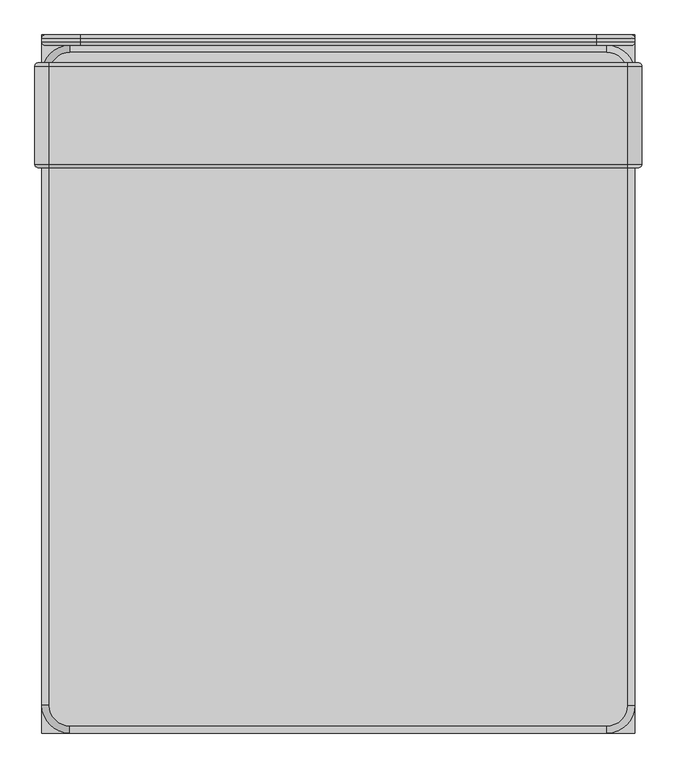
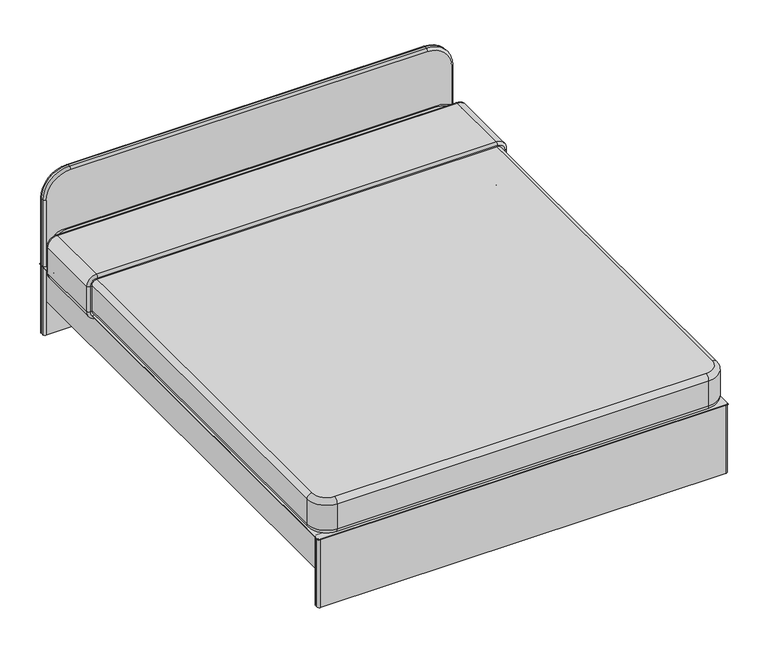
"""IFC4 building model written with IfcOpenShell, lengths in millimetres: furniture geometry, ベッド : 1700 x 2000 mm クィーン."""

from ifc_helpers import new_model, si_unit, point, frame, frame_2d, origin, origin_with_axes, place, context, project, spatial, polyline, circle_curve, ellipse_curve, trimmed, segment, composite_curve, outline, extrude, source, transform, mapped, element, save
from ifc_brep_helpers import plane_surface, cylinder_surface, revolved_surface, advanced_brep


def furniture_6a23a313(model_context):
    return source(origin(), model_context, "Body", "SolidModel", [
        advanced_brep(
        [(850.0, 960.0, 430.0), (850.0, 680.0, 430.0), (830.0, 680.0, 450.0), (830.0, 960.0, 450.0), (860.0, 970.0, 430.0), (830.0, 970.0, 460.0), (870.0, 960.0, 430.0), (830.0, 960.0, 470.0), (870.0, 680.0, 430.0), (830.0, 680.0, 470.0), (860.0, 670.0, 430.0), (830.0, 670.0, 460.0), (850.0, 960.0, 320.0), (850.0, 680.0, 320.0), (860.0, 970.0, 320.0), (870.0, 960.0, 320.0), (870.0, 680.0, 320.0), (860.0, 670.0, 320.0), (830.0, 960.0, 300.0), (830.0, 680.0, 300.0), (830.0, 970.0, 290.0), (830.0, 960.0, 280.0), (830.0, 680.0, 280.0), (830.0, 670.0, 290.0), (-830.0, 960.0, 300.0), (-830.0, 680.0, 300.0), (-830.0, 970.0, 290.0), (-830.0, 960.0, 280.0), (-830.0, 680.0, 280.0), (-830.0, 670.0, 290.0), (-850.0, 960.0, 320.0), (-850.0, 680.0, 320.0), (-860.0, 970.0, 320.0), (-870.0, 960.0, 320.0), (-870.0, 680.0, 320.0), (-860.0, 670.0, 320.0), (-850.0, 960.0, 430.0), (-850.0, 680.0, 430.0), (-860.0, 970.0, 430.0), (-870.0, 960.0, 430.0), (-870.0, 680.0, 430.0), (-860.0, 670.0, 430.0), (-830.0, 960.0, 450.0), (-830.0, 680.0, 450.0), (-830.0, 970.0, 460.0), (-830.0, 960.0, 470.0), (-830.0, 680.0, 470.0), (-830.0, 670.0, 460.0)],
        [
            (0, 1),
            (1, 2, circle_curve(frame((830.0, 680.0, 430.0), z_axis=(0.0, -1.0, 0.0), x_axis=(0.0, 0.0, 1.0)), 20.0)),
            (2, 3),
            (3, 0, circle_curve(frame((830.0, 960.0, 430.0), z_axis=(0.0, 1.0, 0.0), x_axis=(0.0, 0.0, 1.0)), 20.0)),
            (4, 0, circle_curve(frame((860.0, 960.0, 430.0), z_axis=(0.0, 0.0, 1.0), x_axis=(1.0, 0.0, 0.0)), 10.0)),
            (3, 5, circle_curve(frame((830.0, 960.0, 460.0), z_axis=(1.0, 0.0, 0.0), x_axis=(0.0, 0.0, 1.0)), 10.0)),
            (5, 4, circle_curve(frame((830.0, 970.0, 430.0), z_axis=(0.0, 1.0, 0.0), x_axis=(0.0, 0.0, 1.0)), 30.0)),
            (6, 4, circle_curve(frame((860.0, 960.0, 430.0), z_axis=(0.0, 0.0, 1.0), x_axis=(1.0, 0.0, 0.0)), 10.0)),
            (5, 7, circle_curve(frame((830.0, 960.0, 460.0), z_axis=(1.0, 0.0, 0.0), x_axis=(0.0, 0.0, 1.0)), 10.0)),
            (7, 6, circle_curve(frame((830.0, 960.0, 430.0), z_axis=(0.0, 1.0, 0.0), x_axis=(0.0, 0.0, 1.0)), 40.0)),
            (8, 6),
            (7, 9),
            (9, 8, circle_curve(frame((830.0, 680.0, 430.0), z_axis=(0.0, 1.0, 0.0), x_axis=(0.0, 0.0, 1.0)), 40.0)),
            (10, 8, circle_curve(frame((860.0, 680.0, 430.0), z_axis=(0.0, 0.0, 1.0), x_axis=(1.0, 0.0, 0.0)), 10.0)),
            (9, 11, circle_curve(frame((830.0, 680.0, 460.0), z_axis=(1.0, 0.0, 0.0), x_axis=(0.0, 0.0, 1.0)), 10.0)),
            (11, 10, circle_curve(frame((830.0, 670.0, 430.0), z_axis=(0.0, 1.0, 0.0), x_axis=(0.0, 0.0, 1.0)), 30.0)),
            (1, 10, circle_curve(frame((860.0, 680.0, 430.0), z_axis=(0.0, 0.0, 1.0), x_axis=(1.0, 0.0, 0.0)), 10.0)),
            (11, 2, circle_curve(frame((830.0, 680.0, 460.0), z_axis=(1.0, 0.0, 0.0), x_axis=(0.0, 0.0, 1.0)), 10.0)),
            (0, 12),
            (12, 13),
            (13, 1),
            (4, 14),
            (14, 12, circle_curve(frame((860.0, 960.0, 320.0), z_axis=(0.0, 0.0, 1.0), x_axis=(1.0, 0.0, 0.0)), 10.0)),
            (6, 15),
            (15, 14, circle_curve(frame((860.0, 960.0, 320.0), z_axis=(0.0, 0.0, 1.0), x_axis=(1.0, 0.0, 0.0)), 10.0)),
            (8, 16),
            (16, 15),
            (10, 17),
            (17, 16, circle_curve(frame((860.0, 680.0, 320.0), z_axis=(0.0, 0.0, 1.0), x_axis=(1.0, 0.0, 0.0)), 10.0)),
            (13, 17, circle_curve(frame((860.0, 680.0, 320.0), z_axis=(0.0, 0.0, 1.0), x_axis=(1.0, 0.0, 0.0)), 10.0)),
            (18, 19),
            (19, 13, circle_curve(frame((830.0, 680.0, 320.0), z_axis=(0.0, -1.0, 0.0), x_axis=(1.0, 0.0, 0.0)), 20.0)),
            (12, 18, circle_curve(frame((830.0, 960.0, 320.0), z_axis=(0.0, 1.0, 0.0), x_axis=(1.0, 0.0, 0.0)), 20.0)),
            (20, 18, circle_curve(frame((830.0, 960.0, 290.0), z_axis=(1.0, 0.0, 0.0), x_axis=(0.0, 0.0, -1.0)), 10.0)),
            (14, 20, circle_curve(frame((830.0, 970.0, 320.0), z_axis=(0.0, 1.0, 0.0), x_axis=(1.0, 0.0, 0.0)), 30.0)),
            (21, 20, circle_curve(frame((830.0, 960.0, 290.0), z_axis=(1.0, 0.0, 0.0), x_axis=(0.0, 0.0, -1.0)), 10.0)),
            (15, 21, circle_curve(frame((830.0, 960.0, 320.0), z_axis=(0.0, 1.0, 0.0), x_axis=(1.0, 0.0, 0.0)), 40.0)),
            (22, 21),
            (16, 22, circle_curve(frame((830.0, 680.0, 320.0), z_axis=(0.0, 1.0, 0.0), x_axis=(1.0, 0.0, 0.0)), 40.0)),
            (23, 22, circle_curve(frame((830.0, 680.0, 290.0), z_axis=(1.0, 0.0, 0.0), x_axis=(0.0, 0.0, -1.0)), 10.0)),
            (17, 23, circle_curve(frame((830.0, 670.0, 320.0), z_axis=(0.0, 1.0, 0.0), x_axis=(1.0, 0.0, 0.0)), 30.0)),
            (19, 23, circle_curve(frame((830.0, 680.0, 290.0), z_axis=(1.0, 0.0, 0.0), x_axis=(0.0, 0.0, -1.0)), 10.0)),
            (18, 24),
            (24, 25),
            (25, 19),
            (20, 26),
            (26, 24, circle_curve(frame((-830.0, 960.0, 290.0), z_axis=(1.0, 0.0, 0.0), x_axis=(0.0, 0.0, -1.0)), 10.0)),
            (21, 27),
            (27, 26, circle_curve(frame((-830.0, 960.0, 290.0), z_axis=(1.0, 0.0, 0.0), x_axis=(0.0, 0.0, -1.0)), 10.0)),
            (22, 28),
            (28, 27),
            (23, 29),
            (29, 28, circle_curve(frame((-830.0, 680.0, 290.0), z_axis=(1.0, 0.0, 0.0), x_axis=(0.0, 0.0, -1.0)), 10.0)),
            (25, 29, circle_curve(frame((-830.0, 680.0, 290.0), z_axis=(1.0, 0.0, 0.0), x_axis=(0.0, 0.0, -1.0)), 10.0)),
            (30, 31),
            (31, 25, circle_curve(frame((-830.0, 680.0, 320.0), z_axis=(0.0, -1.0, 0.0), x_axis=(0.0, 0.0, -1.0)), 20.0)),
            (24, 30, circle_curve(frame((-830.0, 960.0, 320.0), z_axis=(0.0, 1.0, 0.0), x_axis=(0.0, 0.0, -1.0)), 20.0)),
            (32, 30, circle_curve(frame((-860.0, 960.0, 320.0), z_axis=(0.0, 0.0, -1.0), x_axis=(-1.0, 0.0, 0.0)), 10.0)),
            (26, 32, circle_curve(frame((-830.0, 970.0, 320.0), z_axis=(0.0, 1.0, 0.0), x_axis=(0.0, 0.0, -1.0)), 30.0)),
            (33, 32, circle_curve(frame((-860.0, 960.0, 320.0), z_axis=(0.0, 0.0, -1.0), x_axis=(-1.0, 0.0, 0.0)), 10.0)),
            (27, 33, circle_curve(frame((-830.0, 960.0, 320.0), z_axis=(0.0, 1.0, 0.0), x_axis=(0.0, 0.0, -1.0)), 40.0)),
            (34, 33),
            (28, 34, circle_curve(frame((-830.0, 680.0, 320.0), z_axis=(0.0, 1.0, 0.0), x_axis=(0.0, 0.0, -1.0)), 40.0)),
            (35, 34, circle_curve(frame((-860.0, 680.0, 320.0), z_axis=(0.0, 0.0, -1.0), x_axis=(-1.0, 0.0, 0.0)), 10.0)),
            (29, 35, circle_curve(frame((-830.0, 670.0, 320.0), z_axis=(0.0, 1.0, 0.0), x_axis=(0.0, 0.0, -1.0)), 30.0)),
            (31, 35, circle_curve(frame((-860.0, 680.0, 320.0), z_axis=(0.0, 0.0, -1.0), x_axis=(-1.0, 0.0, 0.0)), 10.0)),
            (30, 36),
            (36, 37),
            (37, 31),
            (32, 38),
            (38, 36, circle_curve(frame((-860.0, 960.0, 430.0), z_axis=(0.0, 0.0, -1.0), x_axis=(-1.0, 0.0, 0.0)), 10.0)),
            (33, 39),
            (39, 38, circle_curve(frame((-860.0, 960.0, 430.0), z_axis=(0.0, 0.0, -1.0), x_axis=(-1.0, 0.0, 0.0)), 10.0)),
            (34, 40),
            (40, 39),
            (35, 41),
            (41, 40, circle_curve(frame((-860.0, 680.0, 430.0), z_axis=(0.0, 0.0, -1.0), x_axis=(-1.0, 0.0, 0.0)), 10.0)),
            (37, 41, circle_curve(frame((-860.0, 680.0, 430.0), z_axis=(0.0, 0.0, -1.0), x_axis=(-1.0, 0.0, 0.0)), 10.0)),
            (42, 43),
            (43, 37, circle_curve(frame((-830.0, 680.0, 430.0), z_axis=(0.0, -1.0, 0.0), x_axis=(-1.0, 0.0, 0.0)), 20.0)),
            (36, 42, circle_curve(frame((-830.0, 960.0, 430.0), z_axis=(0.0, 1.0, 0.0), x_axis=(-1.0, 0.0, 0.0)), 20.0)),
            (44, 42, circle_curve(frame((-830.0, 960.0, 460.0), z_axis=(-1.0, 0.0, 0.0), x_axis=(0.0, 0.0, 1.0)), 10.0)),
            (38, 44, circle_curve(frame((-830.0, 970.0, 430.0), z_axis=(0.0, 1.0, 0.0), x_axis=(-1.0, 0.0, 0.0)), 30.0)),
            (45, 44, circle_curve(frame((-830.0, 960.0, 460.0), z_axis=(-1.0, 0.0, 0.0), x_axis=(0.0, 0.0, 1.0)), 10.0)),
            (39, 45, circle_curve(frame((-830.0, 960.0, 430.0), z_axis=(0.0, 1.0, 0.0), x_axis=(-1.0, 0.0, 0.0)), 40.0)),
            (46, 45),
            (40, 46, circle_curve(frame((-830.0, 680.0, 430.0), z_axis=(0.0, 1.0, 0.0), x_axis=(-1.0, 0.0, 0.0)), 40.0)),
            (47, 46, circle_curve(frame((-830.0, 680.0, 460.0), z_axis=(-1.0, 0.0, 0.0), x_axis=(0.0, 0.0, 1.0)), 10.0)),
            (41, 47, circle_curve(frame((-830.0, 670.0, 430.0), z_axis=(0.0, 1.0, 0.0), x_axis=(-1.0, 0.0, 0.0)), 30.0)),
            (43, 47, circle_curve(frame((-830.0, 680.0, 460.0), z_axis=(-1.0, 0.0, 0.0), x_axis=(0.0, 0.0, 1.0)), 10.0)),
            (42, 3),
            (2, 43),
            (44, 5),
            (45, 7),
            (46, 9),
            (47, 11),
        ],
        [
            revolved_surface(polyline([(830.0, 680.0, 450.0), (830.0, 960.0, 450.0)]), (830.0, 970.0, 430.0), (0.0, -1.0, 0.0)),
            revolved_surface(trimmed(ellipse_curve(frame((830.0, 960.0, 460.0), z_axis=(1.0, 0.0, 0.0), x_axis=(0.0, 0.0, 1.0)), 10.0, 10.0), [point((830.0, 960.0, 450.0))], [point((830.0, 970.0, 460.0))], True, "CARTESIAN"), (830.0, 970.0, 430.0), (0.0, -1.0, 0.0)),
            revolved_surface(trimmed(ellipse_curve(frame((830.0, 960.0, 460.0), z_axis=(1.0, 0.0, 0.0), x_axis=(0.0, 0.0, 1.0)), 10.0, 10.0), [point((830.0, 970.0, 460.0))], [point((830.0, 960.0, 470.0))], True, "CARTESIAN"), (830.0, 970.0, 430.0), (0.0, -1.0, 0.0)),
            cylinder_surface(frame((830.0, 970.0, 430.0), z_axis=(0.0, -1.0, 0.0), x_axis=(0.0, 0.0, 1.0)), 40.0),
            revolved_surface(trimmed(ellipse_curve(frame((830.0, 680.0, 460.0), z_axis=(1.0, 0.0, 0.0), x_axis=(0.0, 0.0, 1.0)), 10.0, 10.0), [point((830.0, 680.0, 470.0))], [point((830.0, 670.0, 460.0))], True, "CARTESIAN"), (830.0, 970.0, 430.0), (0.0, -1.0, 0.0)),
            revolved_surface(trimmed(ellipse_curve(frame((830.0, 680.0, 460.0), z_axis=(1.0, 0.0, 0.0), x_axis=(0.0, 0.0, 1.0)), 10.0, 10.0), [point((830.0, 670.0, 460.0))], [point((830.0, 680.0, 450.0))], True, "CARTESIAN"), (830.0, 970.0, 430.0), (0.0, -1.0, 0.0)),
            plane_surface(frame((850.0, 680.0, 430.0), z_axis=(-1.0, 0.0, 0.0), x_axis=(0.0, 0.0, -1.0))),
            cylinder_surface(frame((860.0, 960.0, 430.0), z_axis=(0.0, 0.0, 1.0), x_axis=(1.0, 0.0, 0.0)), 10.0),
            plane_surface(frame((870.0, 960.0, 430.0), z_axis=(1.0, 0.0, 0.0), x_axis=(0.0, 0.0, -1.0))),
            cylinder_surface(frame((860.0, 680.0, 430.0), z_axis=(0.0, 0.0, 1.0), x_axis=(1.0, 0.0, 0.0)), 10.0),
            revolved_surface(polyline([(850.0, 680.0, 320.0), (850.0, 960.0, 320.0)]), (830.0, 970.0, 320.0), (0.0, -1.0, 0.0)),
            revolved_surface(trimmed(ellipse_curve(frame((860.0, 960.0, 320.0), z_axis=(0.0, 0.0, -1.0), x_axis=(1.0, 0.0, 0.0)), 10.0, 10.0), [point((850.0, 960.0, 320.0))], [point((860.0, 970.0, 320.0))], True, "CARTESIAN"), (830.0, 970.0, 320.0), (0.0, -1.0, 0.0)),
            revolved_surface(trimmed(ellipse_curve(frame((860.0, 960.0, 320.0), z_axis=(0.0, 0.0, -1.0), x_axis=(1.0, 0.0, 0.0)), 10.0, 10.0), [point((860.0, 970.0, 320.0))], [point((870.0, 960.0, 320.0))], True, "CARTESIAN"), (830.0, 970.0, 320.0), (0.0, -1.0, 0.0)),
            cylinder_surface(frame((830.0, 970.0, 320.0), z_axis=(0.0, -1.0, 0.0), x_axis=(1.0, 0.0, 0.0)), 40.0),
            revolved_surface(trimmed(ellipse_curve(frame((860.0, 680.0, 320.0), z_axis=(0.0, 0.0, -1.0), x_axis=(1.0, 0.0, 0.0)), 10.0, 10.0), [point((870.0, 680.0, 320.0))], [point((860.0, 670.0, 320.0))], True, "CARTESIAN"), (830.0, 970.0, 320.0), (0.0, -1.0, 0.0)),
            revolved_surface(trimmed(ellipse_curve(frame((860.0, 680.0, 320.0), z_axis=(0.0, 0.0, -1.0), x_axis=(1.0, 0.0, 0.0)), 10.0, 10.0), [point((860.0, 670.0, 320.0))], [point((850.0, 680.0, 320.0))], True, "CARTESIAN"), (830.0, 970.0, 320.0), (0.0, -1.0, 0.0)),
            plane_surface(frame((830.0, 680.0, 300.0), z_axis=(0.0, 0.0, 1.0), x_axis=(-1.0, 0.0, 0.0))),
            cylinder_surface(frame((830.0, 960.0, 290.0), z_axis=(1.0, 0.0, 0.0), x_axis=(0.0, 0.0, -1.0)), 10.0),
            plane_surface(frame((830.0, 960.0, 280.0), z_axis=(0.0, 0.0, -1.0), x_axis=(-1.0, 0.0, 0.0))),
            cylinder_surface(frame((830.0, 680.0, 290.0), z_axis=(1.0, 0.0, 0.0), x_axis=(0.0, 0.0, -1.0)), 10.0),
            revolved_surface(polyline([(-830.0, 680.0, 300.0), (-830.0, 960.0, 300.0)]), (-830.0, 970.0, 320.0), (0.0, -1.0, 0.0)),
            revolved_surface(trimmed(ellipse_curve(frame((-830.0, 960.0, 290.0), z_axis=(-1.0, 0.0, 0.0), x_axis=(0.0, 0.0, -1.0)), 10.0, 10.0), [point((-830.0, 960.0, 300.0))], [point((-830.0, 970.0, 290.0))], True, "CARTESIAN"), (-830.0, 970.0, 320.0), (0.0, -1.0, 0.0)),
            revolved_surface(trimmed(ellipse_curve(frame((-830.0, 960.0, 290.0), z_axis=(-1.0, 0.0, 0.0), x_axis=(0.0, 0.0, -1.0)), 10.0, 10.0), [point((-830.0, 970.0, 290.0))], [point((-830.0, 960.0, 280.0))], True, "CARTESIAN"), (-830.0, 970.0, 320.0), (0.0, -1.0, 0.0)),
            cylinder_surface(frame((-830.0, 970.0, 320.0), z_axis=(0.0, -1.0, 0.0), x_axis=(0.0, 0.0, -1.0)), 40.0),
            revolved_surface(trimmed(ellipse_curve(frame((-830.0, 680.0, 290.0), z_axis=(-1.0, 0.0, 0.0), x_axis=(0.0, 0.0, -1.0)), 10.0, 10.0), [point((-830.0, 680.0, 280.0))], [point((-830.0, 670.0, 290.0))], True, "CARTESIAN"), (-830.0, 970.0, 320.0), (0.0, -1.0, 0.0)),
            revolved_surface(trimmed(ellipse_curve(frame((-830.0, 680.0, 290.0), z_axis=(-1.0, 0.0, 0.0), x_axis=(0.0, 0.0, -1.0)), 10.0, 10.0), [point((-830.0, 670.0, 290.0))], [point((-830.0, 680.0, 300.0))], True, "CARTESIAN"), (-830.0, 970.0, 320.0), (0.0, -1.0, 0.0)),
            plane_surface(frame((-850.0, 680.0, 320.0), z_axis=(1.0, 0.0, 0.0), x_axis=(0.0, 0.0, 1.0))),
            cylinder_surface(frame((-860.0, 960.0, 320.0), z_axis=(0.0, 0.0, -1.0), x_axis=(-1.0, 0.0, 0.0)), 10.0),
            plane_surface(frame((-870.0, 960.0, 320.0), z_axis=(-1.0, 0.0, 0.0), x_axis=(0.0, 0.0, 1.0))),
            cylinder_surface(frame((-860.0, 680.0, 320.0), z_axis=(0.0, 0.0, -1.0), x_axis=(-1.0, 0.0, 0.0)), 10.0),
            revolved_surface(polyline([(-850.0, 680.0, 430.0), (-850.0, 960.0, 430.0)]), (-830.0, 970.0, 430.0), (0.0, -1.0, 0.0)),
            revolved_surface(trimmed(ellipse_curve(frame((-860.0, 960.0, 430.0), z_axis=(0.0, 0.0, 1.0), x_axis=(-1.0, 0.0, 0.0)), 10.0, 10.0), [point((-850.0, 960.0, 430.0))], [point((-860.0, 970.0, 430.0))], True, "CARTESIAN"), (-830.0, 970.0, 430.0), (0.0, -1.0, 0.0)),
            revolved_surface(trimmed(ellipse_curve(frame((-860.0, 960.0, 430.0), z_axis=(0.0, 0.0, 1.0), x_axis=(-1.0, 0.0, 0.0)), 10.0, 10.0), [point((-860.0, 970.0, 430.0))], [point((-870.0, 960.0, 430.0))], True, "CARTESIAN"), (-830.0, 970.0, 430.0), (0.0, -1.0, 0.0)),
            cylinder_surface(frame((-830.0, 970.0, 430.0), z_axis=(0.0, -1.0, 0.0), x_axis=(-1.0, 0.0, 0.0)), 40.0),
            revolved_surface(trimmed(ellipse_curve(frame((-860.0, 680.0, 430.0), z_axis=(0.0, 0.0, 1.0), x_axis=(-1.0, 0.0, 0.0)), 10.0, 10.0), [point((-870.0, 680.0, 430.0))], [point((-860.0, 670.0, 430.0))], True, "CARTESIAN"), (-830.0, 970.0, 430.0), (0.0, -1.0, 0.0)),
            revolved_surface(trimmed(ellipse_curve(frame((-860.0, 680.0, 430.0), z_axis=(0.0, 0.0, 1.0), x_axis=(-1.0, 0.0, 0.0)), 10.0, 10.0), [point((-860.0, 670.0, 430.0))], [point((-850.0, 680.0, 430.0))], True, "CARTESIAN"), (-830.0, 970.0, 430.0), (0.0, -1.0, 0.0)),
            plane_surface(frame((-830.0, 680.0, 450.0), z_axis=(0.0, 0.0, -1.0), x_axis=(1.0, 0.0, 0.0))),
            cylinder_surface(frame((-830.0, 960.0, 460.0), z_axis=(-1.0, 0.0, 0.0), x_axis=(0.0, 0.0, 1.0)), 10.0),
            plane_surface(frame((-830.0, 960.0, 470.0), z_axis=(0.0, 0.0, 1.0), x_axis=(1.0, 0.0, 0.0))),
            cylinder_surface(frame((-830.0, 680.0, 460.0), z_axis=(-1.0, 0.0, 0.0), x_axis=(0.0, 0.0, 1.0)), 10.0),
        ],
        [
            (0, [[1, 2, 3, 4]]),
            (1, [[5, -4, 6, 7]]),
            (2, [[8, -7, 9, 10]]),
            (3, [[11, -10, 12, 13]]),
            (4, [[14, -13, 15, 16]]),
            (5, [[17, -16, 18, -2]]),
            (6, [[19, 20, 21, -1]]),
            (7, [[22, 23, -19, -5]]),
            (7, [[24, 25, -22, -8]]),
            (8, [[26, 27, -24, -11]]),
            (9, [[28, 29, -26, -14]]),
            (9, [[-21, 30, -28, -17]]),
            (10, [[31, 32, -20, 33]]),
            (11, [[34, -33, -23, 35]]),
            (12, [[36, -35, -25, 37]]),
            (13, [[38, -37, -27, 39]]),
            (14, [[40, -39, -29, 41]]),
            (15, [[42, -41, -30, -32]]),
            (16, [[43, 44, 45, -31]]),
            (17, [[46, 47, -43, -34]]),
            (17, [[48, 49, -46, -36]]),
            (18, [[50, 51, -48, -38]]),
            (19, [[52, 53, -50, -40]]),
            (19, [[-45, 54, -52, -42]]),
            (20, [[55, 56, -44, 57]]),
            (21, [[58, -57, -47, 59]]),
            (22, [[60, -59, -49, 61]]),
            (23, [[62, -61, -51, 63]]),
            (24, [[64, -63, -53, 65]]),
            (25, [[66, -65, -54, -56]]),
            (26, [[67, 68, 69, -55]]),
            (27, [[70, 71, -67, -58]]),
            (27, [[72, 73, -70, -60]]),
            (28, [[74, 75, -72, -62]]),
            (29, [[76, 77, -74, -64]]),
            (29, [[-69, 78, -76, -66]]),
            (30, [[79, 80, -68, 81]]),
            (31, [[82, -81, -71, 83]]),
            (32, [[84, -83, -73, 85]]),
            (33, [[86, -85, -75, 87]]),
            (34, [[88, -87, -77, 89]]),
            (35, [[90, -89, -78, -80]]),
            (36, [[91, -3, 92, -79]]),
            (37, [[93, -6, -91, -82]]),
            (37, [[94, -9, -93, -84]]),
            (38, [[95, -12, -94, -86]]),
            (39, [[96, -15, -95, -88]]),
            (39, [[-92, -18, -96, -90]]),
        ],
    ),
        extrude(outline(polyline([(850.0, 1050.0), (850.0, -950.0), (-850.0, -950.0), (-850.0, 1050.0), (850.0, 1050.0)])), frame((0.0, 0.0, 298.0), z_axis=(0.0, 0.0, 1.0), x_axis=(1.0, 0.0, 0.0)), (0.0, 0.0, 1.0), 2.0),
        advanced_brep(
        [(850.0, 940.0, 320.0), (830.0, 940.0, 300.0), (770.0, 1000.0, 300.0), (770.0, 1020.0, 320.0), (770.0, 1020.0, 430.0), (850.0, 940.0, 430.0), (770.0, 1000.0, 450.0), (830.0, 940.0, 450.0), (850.0, -870.0, 320.0), (830.0, -870.0, 300.0), (850.0, -870.0, 430.0), (830.0, -870.0, 450.0), (770.0, -950.0, 320.0), (770.0, -930.0, 300.0), (770.0, -950.0, 430.0), (770.0, -930.0, 450.0), (-770.0, -950.0, 320.0), (-770.0, -930.0, 300.0), (-770.0, -950.0, 430.0), (-770.0, -930.0, 450.0), (-850.0, -870.0, 320.0), (-830.0, -870.0, 300.0), (-850.0, -870.0, 430.0), (-830.0, -870.0, 450.0), (-850.0, 940.0, 320.0), (-830.0, 940.0, 300.0), (-850.0, 940.0, 430.0), (-830.0, 940.0, 450.0), (-770.0, 1020.0, 320.0), (-770.0, 1000.0, 300.0), (-770.0, 1020.0, 430.0), (-770.0, 1000.0, 450.0)],
        [
            (0, 1, circle_curve(frame((830.0, 940.0, 320.0), z_axis=(0.0, 1.0, 0.0), x_axis=(-1.0, 0.0, 0.0)), 20.0)),
            (1, 2, circle_curve(frame((770.0, 940.0, 300.0), z_axis=(0.0, 0.0, 1.0), x_axis=(0.0, 1.0, 0.0)), 60.0)),
            (2, 3, circle_curve(frame((770.0, 1000.0, 320.0), z_axis=(1.0, 0.0, 0.0), x_axis=(0.0, -1.0, 0.0)), 20.0)),
            (3, 0, circle_curve(frame((770.0, 940.0, 320.0), z_axis=(0.0, 0.0, -1.0), x_axis=(0.0, 1.0, 0.0)), 80.0)),
            (3, 4),
            (4, 5, circle_curve(frame((770.0, 940.0, 430.0), z_axis=(0.0, 0.0, -1.0), x_axis=(0.0, 1.0, 0.0)), 80.0)),
            (5, 0),
            (4, 6, circle_curve(frame((770.0, 1000.0, 430.0), z_axis=(1.0, 0.0, 0.0), x_axis=(0.0, -1.0, 0.0)), 20.0)),
            (6, 7, circle_curve(frame((770.0, 940.0, 450.0), z_axis=(0.0, 0.0, -1.0), x_axis=(0.0, 1.0, 0.0)), 60.0)),
            (7, 5, circle_curve(frame((830.0, 940.0, 430.0), z_axis=(0.0, 1.0, 0.0), x_axis=(-1.0, 0.0, 0.0)), 20.0)),
            (0, 8),
            (8, 9, circle_curve(frame((830.0, -870.0, 320.0), z_axis=(0.0, 1.0, 0.0), x_axis=(-1.0, 0.0, 0.0)), 20.0)),
            (9, 1),
            (5, 10),
            (10, 8),
            (7, 11),
            (11, 10, circle_curve(frame((830.0, -870.0, 430.0), z_axis=(0.0, 1.0, 0.0), x_axis=(-1.0, 0.0, 0.0)), 20.0)),
            (8, 12, circle_curve(frame((770.0, -870.0, 320.0), z_axis=(0.0, 0.0, -1.0), x_axis=(1.0, 0.0, 0.0)), 80.0)),
            (12, 13, circle_curve(frame((770.0, -930.0, 320.0), z_axis=(1.0, 0.0, 0.0), x_axis=(0.0, 1.0, 0.0)), 20.0)),
            (13, 9, circle_curve(frame((770.0, -870.0, 300.0), z_axis=(0.0, 0.0, 1.0), x_axis=(1.0, 0.0, 0.0)), 60.0)),
            (10, 14, circle_curve(frame((770.0, -870.0, 430.0), z_axis=(0.0, 0.0, -1.0), x_axis=(1.0, 0.0, 0.0)), 80.0)),
            (14, 12),
            (11, 15, circle_curve(frame((770.0, -870.0, 450.0), z_axis=(0.0, 0.0, -1.0), x_axis=(1.0, 0.0, 0.0)), 60.0)),
            (15, 14, circle_curve(frame((770.0, -930.0, 430.0), z_axis=(1.0, 0.0, 0.0), x_axis=(0.0, 1.0, 0.0)), 20.0)),
            (12, 16),
            (16, 17, circle_curve(frame((-770.0, -930.0, 320.0), z_axis=(1.0, 0.0, 0.0), x_axis=(0.0, 1.0, 0.0)), 20.0)),
            (17, 13),
            (14, 18),
            (18, 16),
            (15, 19),
            (19, 18, circle_curve(frame((-770.0, -930.0, 430.0), z_axis=(1.0, 0.0, 0.0), x_axis=(0.0, 1.0, 0.0)), 20.0)),
            (16, 20, circle_curve(frame((-770.0, -870.0, 320.0), z_axis=(0.0, 0.0, -1.0), x_axis=(0.0, -1.0, 0.0)), 80.0)),
            (20, 21, circle_curve(frame((-830.0, -870.0, 320.0), z_axis=(0.0, -1.0, 0.0), x_axis=(1.0, 0.0, 0.0)), 20.0)),
            (21, 17, circle_curve(frame((-770.0, -870.0, 300.0), z_axis=(0.0, 0.0, 1.0), x_axis=(0.0, -1.0, 0.0)), 60.0)),
            (18, 22, circle_curve(frame((-770.0, -870.0, 430.0), z_axis=(0.0, 0.0, -1.0), x_axis=(0.0, -1.0, 0.0)), 80.0)),
            (22, 20),
            (19, 23, circle_curve(frame((-770.0, -870.0, 450.0), z_axis=(0.0, 0.0, -1.0), x_axis=(0.0, -1.0, 0.0)), 60.0)),
            (23, 22, circle_curve(frame((-830.0, -870.0, 430.0), z_axis=(0.0, -1.0, 0.0), x_axis=(1.0, 0.0, 0.0)), 20.0)),
            (20, 24),
            (24, 25, circle_curve(frame((-830.0, 940.0, 320.0), z_axis=(0.0, -1.0, 0.0), x_axis=(1.0, 0.0, 0.0)), 20.0)),
            (25, 21),
            (22, 26),
            (26, 24),
            (23, 27),
            (27, 26, circle_curve(frame((-830.0, 940.0, 430.0), z_axis=(0.0, -1.0, 0.0), x_axis=(1.0, 0.0, 0.0)), 20.0)),
            (24, 28, circle_curve(frame((-770.0, 940.0, 320.0), z_axis=(0.0, 0.0, -1.0), x_axis=(-1.0, 0.0, 0.0)), 80.0)),
            (28, 29, circle_curve(frame((-770.0, 1000.0, 320.0), z_axis=(-1.0, 0.0, 0.0), x_axis=(0.0, -1.0, 0.0)), 20.0)),
            (29, 25, circle_curve(frame((-770.0, 940.0, 300.0), z_axis=(0.0, 0.0, 1.0), x_axis=(-1.0, 0.0, 0.0)), 60.0)),
            (26, 30, circle_curve(frame((-770.0, 940.0, 430.0), z_axis=(0.0, 0.0, -1.0), x_axis=(-1.0, 0.0, 0.0)), 80.0)),
            (30, 28),
            (27, 31, circle_curve(frame((-770.0, 940.0, 450.0), z_axis=(0.0, 0.0, -1.0), x_axis=(-1.0, 0.0, 0.0)), 60.0)),
            (31, 30, circle_curve(frame((-770.0, 1000.0, 430.0), z_axis=(-1.0, 0.0, 0.0), x_axis=(0.0, -1.0, 0.0)), 20.0)),
            (6, 31),
            (29, 2),
            (28, 3),
            (30, 4),
        ],
        [
            revolved_surface(trimmed(ellipse_curve(frame((770.0, 1000.0, 320.0), z_axis=(1.0, 0.0, 0.0), x_axis=(0.0, -1.0, 0.0)), 20.0, 20.0), [point((770.0, 1000.0, 300.0))], [point((770.0, 1020.0, 320.0))], True, "CARTESIAN"), (770.0, 940.0, 300.0), (0.0, 0.0, 1.0)),
            cylinder_surface(frame((770.0, 940.0, 300.0), z_axis=(0.0, 0.0, 1.0), x_axis=(0.0, 1.0, 0.0)), 80.0),
            revolved_surface(trimmed(ellipse_curve(frame((770.0, 1000.0, 430.0), z_axis=(1.0, 0.0, 0.0), x_axis=(0.0, -1.0, 0.0)), 20.0, 20.0), [point((770.0, 1020.0, 430.0))], [point((770.0, 1000.0, 450.0))], True, "CARTESIAN"), (770.0, 940.0, 300.0), (0.0, 0.0, 1.0)),
            cylinder_surface(frame((830.0, 940.0, 320.0), z_axis=(0.0, 1.0, 0.0), x_axis=(-1.0, 0.0, 0.0)), 20.0),
            plane_surface(frame((850.0, 940.0, 320.0), z_axis=(1.0, 0.0, 0.0), x_axis=(0.0, -1.0, 0.0))),
            cylinder_surface(frame((830.0, 940.0, 430.0), z_axis=(0.0, 1.0, 0.0), x_axis=(-1.0, 0.0, 0.0)), 20.0),
            revolved_surface(trimmed(ellipse_curve(frame((830.0, -870.0, 320.0), z_axis=(0.0, -1.0, 0.0), x_axis=(-1.0, 0.0, 0.0)), 20.0, 20.0), [point((830.0, -870.0, 300.0))], [point((850.0, -870.0, 320.0))], True, "CARTESIAN"), (770.0, -870.0, 300.0), (0.0, 0.0, 1.0)),
            cylinder_surface(frame((770.0, -870.0, 300.0), z_axis=(0.0, 0.0, 1.0), x_axis=(1.0, 0.0, 0.0)), 80.0),
            revolved_surface(trimmed(ellipse_curve(frame((830.0, -870.0, 430.0), z_axis=(0.0, -1.0, 0.0), x_axis=(-1.0, 0.0, 0.0)), 20.0, 20.0), [point((850.0, -870.0, 430.0))], [point((830.0, -870.0, 450.0))], True, "CARTESIAN"), (770.0, -870.0, 300.0), (0.0, 0.0, 1.0)),
            cylinder_surface(frame((770.0, -930.0, 320.0), z_axis=(1.0, 0.0, 0.0), x_axis=(0.0, 1.0, 0.0)), 20.0),
            plane_surface(frame((770.0, -950.0, 320.0), z_axis=(0.0, -1.0, 0.0), x_axis=(-1.0, 0.0, 0.0))),
            cylinder_surface(frame((770.0, -930.0, 430.0), z_axis=(1.0, 0.0, 0.0), x_axis=(0.0, 1.0, 0.0)), 20.0),
            revolved_surface(trimmed(ellipse_curve(frame((-770.0, -930.0, 320.0), z_axis=(-1.0, 0.0, 0.0), x_axis=(0.0, 1.0, 0.0)), 20.0, 20.0), [point((-770.0, -930.0, 300.0))], [point((-770.0, -950.0, 320.0))], True, "CARTESIAN"), (-770.0, -870.0, 300.0), (0.0, 0.0, 1.0)),
            cylinder_surface(frame((-770.0, -870.0, 300.0), z_axis=(0.0, 0.0, 1.0), x_axis=(0.0, -1.0, 0.0)), 80.0),
            revolved_surface(trimmed(ellipse_curve(frame((-770.0, -930.0, 430.0), z_axis=(-1.0, 0.0, 0.0), x_axis=(0.0, 1.0, 0.0)), 20.0, 20.0), [point((-770.0, -950.0, 430.0))], [point((-770.0, -930.0, 450.0))], True, "CARTESIAN"), (-770.0, -870.0, 300.0), (0.0, 0.0, 1.0)),
            cylinder_surface(frame((-830.0, -870.0, 320.0), z_axis=(0.0, -1.0, 0.0), x_axis=(1.0, 0.0, 0.0)), 20.0),
            plane_surface(frame((-850.0, -870.0, 320.0), z_axis=(-1.0, 0.0, 0.0), x_axis=(0.0, 1.0, 0.0))),
            cylinder_surface(frame((-830.0, -870.0, 430.0), z_axis=(0.0, -1.0, 0.0), x_axis=(1.0, 0.0, 0.0)), 20.0),
            revolved_surface(trimmed(ellipse_curve(frame((-830.0, 940.0, 320.0), z_axis=(0.0, 1.0, 0.0), x_axis=(1.0, 0.0, 0.0)), 20.0, 20.0), [point((-830.0, 940.0, 300.0))], [point((-850.0, 940.0, 320.0))], True, "CARTESIAN"), (-770.0, 940.0, 300.0), (0.0, 0.0, 1.0)),
            cylinder_surface(frame((-770.0, 940.0, 300.0), z_axis=(0.0, 0.0, 1.0), x_axis=(-1.0, 0.0, 0.0)), 80.0),
            revolved_surface(trimmed(ellipse_curve(frame((-830.0, 940.0, 430.0), z_axis=(0.0, 1.0, 0.0), x_axis=(1.0, 0.0, 0.0)), 20.0, 20.0), [point((-850.0, 940.0, 430.0))], [point((-830.0, 940.0, 450.0))], True, "CARTESIAN"), (-770.0, 940.0, 300.0), (0.0, 0.0, 1.0)),
            plane_surface(frame((-770.0, 940.0, 450.0), z_axis=(0.0, 0.0, 1.0), x_axis=(-1.0, 0.0, 0.0))),
            plane_surface(frame((-770.0, 940.0, 300.0), z_axis=(0.0, 0.0, -1.0), x_axis=(-1.0, 0.0, 0.0))),
            cylinder_surface(frame((-770.0, 1000.0, 320.0), z_axis=(-1.0, 0.0, 0.0), x_axis=(0.0, -1.0, 0.0)), 20.0),
            plane_surface(frame((-770.0, 1020.0, 320.0), z_axis=(0.0, 1.0, 0.0), x_axis=(1.0, 0.0, 0.0))),
            cylinder_surface(frame((-770.0, 1000.0, 430.0), z_axis=(-1.0, 0.0, 0.0), x_axis=(0.0, -1.0, 0.0)), 20.0),
        ],
        [
            (0, [[1, 2, 3, 4]]),
            (1, [[5, 6, 7, -4]]),
            (2, [[8, 9, 10, -6]]),
            (3, [[11, 12, 13, -1]]),
            (4, [[14, 15, -11, -7]]),
            (5, [[16, 17, -14, -10]]),
            (6, [[18, 19, 20, -12]]),
            (7, [[21, 22, -18, -15]]),
            (8, [[23, 24, -21, -17]]),
            (9, [[25, 26, 27, -19]]),
            (10, [[28, 29, -25, -22]]),
            (11, [[30, 31, -28, -24]]),
            (12, [[32, 33, 34, -26]]),
            (13, [[35, 36, -32, -29]]),
            (14, [[37, 38, -35, -31]]),
            (15, [[39, 40, 41, -33]]),
            (16, [[42, 43, -39, -36]]),
            (17, [[44, 45, -42, -38]]),
            (18, [[46, 47, 48, -40]]),
            (19, [[49, 50, -46, -43]]),
            (20, [[51, 52, -49, -45]]),
            (21, [[53, -51, -44, -37, -30, -23, -16, -9]]),
            (22, [[-13, -20, -27, -34, -41, -48, 54, -2]]),
            (23, [[-54, -47, 55, -3]]),
            (24, [[-55, -50, 56, -5]]),
            (25, [[-56, -52, -53, -8]]),
        ],
    ),
        extrude(outline(polyline([(840.0, 1020.0), (840.0, -920.0), (-840.0, -920.0), (-840.0, 1020.0), (840.0, 1020.0)])), frame((0.0, 0.0, 150.0), z_axis=(0.0, 0.0, 1.0), x_axis=(1.0, 0.0, 0.0)), (0.0, 0.0, 1.0), 150.0),
        extrude(outline(composite_curve([segment(polyline([(840.0, -950.0), (-840.0, -950.0)]), True, "CONTINUOUS"), segment(trimmed(circle_curve(frame_2d((-840.0, -940.0)), 10.0), [point((-840.0, -950.0))], [point((-850.0, -940.0))], False, "CARTESIAN"), True, "CONTINUOUS"), segment(polyline([(-850.0, -940.0), (-850.0, -930.0)]), True, "CONTINUOUS"), segment(trimmed(circle_curve(frame_2d((-840.0, -930.0)), 10.0), [point((-850.0, -930.0))], [point((-840.0, -920.0))], False, "CARTESIAN"), True, "CONTINUOUS"), segment(polyline([(-840.0, -920.0), (840.0, -920.0)]), True, "CONTINUOUS"), segment(trimmed(circle_curve(frame_2d((840.0, -930.0)), 10.0), [point((840.0, -920.0))], [point((850.0, -930.0))], False, "CARTESIAN"), True, "CONTINUOUS"), segment(polyline([(850.0, -930.0), (850.0, -940.0)]), True, "CONTINUOUS"), segment(trimmed(circle_curve(frame_2d((840.0, -940.0)), 10.0), [point((850.0, -940.0))], [point((840.0, -950.0))], False, "CARTESIAN"), True, "CONTINUOUS")], self_intersect=False)), origin_with_axes(), (0.0, 0.0, 1.0), 300.0),
        advanced_brep(
        [(-840.0, 1050.0, 0.0), (840.0, 1050.0, 0.0), (850.0, 1040.0, 0.0), (850.0, 1030.0, 0.0), (840.0, 1020.0, 0.0), (-840.0, 1020.0, 0.0), (-850.0, 1030.0, 0.0), (-850.0, 1040.0, 0.0), (-840.0, 1050.0, 590.0), (-740.0, 1050.0, 690.0), (740.0, 1050.0, 690.0), (840.0, 1050.0, 590.0), (-850.0, 1040.0, 590.0), (-850.0, 1030.0, 590.0), (-840.0, 1020.0, 590.0), (840.0, 1020.0, 590.0), (740.0, 1020.0, 690.0), (-740.0, 1020.0, 690.0), (-740.0, 1040.0, 700.0), (-740.0, 1030.0, 700.0), (740.0, 1040.0, 700.0), (740.0, 1030.0, 700.0), (850.0, 1040.0, 590.0), (850.0, 1030.0, 590.0)],
        [
            (0, 1),
            (1, 2, circle_curve(frame((840.0, 1040.0, 0.0), z_axis=(0.0, 0.0, -1.0), x_axis=(1.0, 0.0, 0.0)), 10.0)),
            (2, 3),
            (3, 4, circle_curve(frame((840.0, 1030.0, 0.0), z_axis=(0.0, 0.0, -1.0), x_axis=(1.0, 0.0, 0.0)), 10.0)),
            (4, 5),
            (5, 6, circle_curve(frame((-840.0, 1030.0, 0.0), z_axis=(0.0, 0.0, -1.0), x_axis=(-1.0, 0.0, 0.0)), 10.0)),
            (6, 7),
            (7, 0, circle_curve(frame((-840.0, 1040.0, 0.0), z_axis=(0.0, 0.0, -1.0), x_axis=(-1.0, 0.0, 0.0)), 10.0)),
            (0, 8),
            (8, 9, circle_curve(frame((-740.0, 1050.0, 590.0), z_axis=(0.0, 1.0, 0.0), x_axis=(-1.0, 0.0, 0.0)), 100.0)),
            (9, 10),
            (10, 11, circle_curve(frame((740.0, 1050.0, 590.0), z_axis=(0.0, 1.0, 0.0), x_axis=(0.0, 0.0, 1.0)), 100.0)),
            (11, 1),
            (7, 12),
            (12, 8, circle_curve(frame((-840.0, 1040.0, 590.0), z_axis=(0.0, 0.0, -1.0), x_axis=(-1.0, 0.0, 0.0)), 10.0)),
            (6, 13),
            (13, 12),
            (5, 14),
            (14, 13, circle_curve(frame((-840.0, 1030.0, 590.0), z_axis=(0.0, 0.0, -1.0), x_axis=(-1.0, 0.0, 0.0)), 10.0)),
            (4, 15),
            (15, 16, circle_curve(frame((740.0, 1020.0, 590.0), z_axis=(0.0, -1.0, 0.0), x_axis=(0.0, 0.0, 1.0)), 100.0)),
            (16, 17),
            (17, 14, circle_curve(frame((-740.0, 1020.0, 590.0), z_axis=(0.0, -1.0, 0.0), x_axis=(-1.0, 0.0, 0.0)), 100.0)),
            (12, 18, circle_curve(frame((-740.0, 1040.0, 590.0), z_axis=(0.0, 1.0, 0.0), x_axis=(-1.0, 0.0, 0.0)), 110.0)),
            (18, 9, circle_curve(frame((-740.0, 1040.0, 690.0), z_axis=(-1.0, 0.0, 0.0), x_axis=(0.0, 0.0, 1.0)), 10.0)),
            (13, 19, circle_curve(frame((-740.0, 1030.0, 590.0), z_axis=(0.0, 1.0, 0.0), x_axis=(-1.0, 0.0, 0.0)), 110.0)),
            (19, 18),
            (17, 19, circle_curve(frame((-740.0, 1030.0, 690.0), z_axis=(-1.0, 0.0, 0.0), x_axis=(0.0, 0.0, 1.0)), 10.0)),
            (18, 20),
            (20, 10, circle_curve(frame((740.0, 1040.0, 690.0), z_axis=(-1.0, 0.0, 0.0), x_axis=(0.0, 0.0, 1.0)), 10.0)),
            (19, 21),
            (21, 20),
            (16, 21, circle_curve(frame((740.0, 1030.0, 690.0), z_axis=(-1.0, 0.0, 0.0), x_axis=(0.0, 0.0, 1.0)), 10.0)),
            (20, 22, circle_curve(frame((740.0, 1040.0, 590.0), z_axis=(0.0, 1.0, 0.0), x_axis=(0.0, 0.0, 1.0)), 110.0)),
            (22, 11, circle_curve(frame((840.0, 1040.0, 590.0), z_axis=(0.0, 0.0, 1.0), x_axis=(1.0, 0.0, 0.0)), 10.0)),
            (21, 23, circle_curve(frame((740.0, 1030.0, 590.0), z_axis=(0.0, 1.0, 0.0), x_axis=(0.0, 0.0, 1.0)), 110.0)),
            (23, 22),
            (15, 23, circle_curve(frame((840.0, 1030.0, 590.0), z_axis=(0.0, 0.0, 1.0), x_axis=(1.0, 0.0, 0.0)), 10.0)),
            (22, 2),
            (23, 3),
        ],
        [
            plane_surface(frame((-790.0, 1113.2455532, 0.0), z_axis=(0.0, 0.0, -1.0), x_axis=(1.0, 0.0, 0.0))),
            plane_surface(frame((-790.0, 1050.0, 0.0), z_axis=(0.0, 1.0, 0.0), x_axis=(0.0, 0.0, 1.0))),
            cylinder_surface(frame((-840.0, 1040.0, 0.0), z_axis=(0.0, 0.0, -1.0), x_axis=(-1.0, 0.0, 0.0)), 10.0),
            plane_surface(frame((-850.0, 1040.0, 0.0), z_axis=(-1.0, 0.0, 0.0), x_axis=(0.0, 0.0, 1.0))),
            cylinder_surface(frame((-840.0, 1030.0, 0.0), z_axis=(0.0, 0.0, -1.0), x_axis=(-1.0, 0.0, 0.0)), 10.0),
            plane_surface(frame((-840.0, 1020.0, 0.0), z_axis=(0.0, -1.0, 0.0), x_axis=(0.0, 0.0, 1.0))),
            revolved_surface(trimmed(ellipse_curve(frame((-840.0, 1040.0, 590.0), z_axis=(0.0, 0.0, 1.0), x_axis=(-1.0, 0.0, 0.0)), 10.0, 10.0), [point((-840.0, 1050.0, 590.0))], [point((-850.0, 1040.0, 590.0))], True, "CARTESIAN"), (-740.0, 1050.0, 590.0), (0.0, -1.0, 0.0)),
            cylinder_surface(frame((-740.0, 1050.0, 590.0), z_axis=(0.0, -1.0, 0.0), x_axis=(-1.0, 0.0, 0.0)), 110.0),
            revolved_surface(trimmed(ellipse_curve(frame((-840.0, 1030.0, 590.0), z_axis=(0.0, 0.0, 1.0), x_axis=(-1.0, 0.0, 0.0)), 10.0, 10.0), [point((-850.0, 1030.0, 590.0))], [point((-840.0, 1020.0, 590.0))], True, "CARTESIAN"), (-740.0, 1050.0, 590.0), (0.0, -1.0, 0.0)),
            cylinder_surface(frame((-740.0, 1040.0, 690.0), z_axis=(-1.0, 0.0, 0.0), x_axis=(0.0, 0.0, 1.0)), 10.0),
            plane_surface(frame((-740.0, 1040.0, 700.0), z_axis=(0.0, 0.0, 1.0), x_axis=(1.0, 0.0, 0.0))),
            cylinder_surface(frame((-740.0, 1030.0, 690.0), z_axis=(-1.0, 0.0, 0.0), x_axis=(0.0, 0.0, 1.0)), 10.0),
            revolved_surface(trimmed(ellipse_curve(frame((740.0, 1040.0, 690.0), z_axis=(1.0, 0.0, 0.0), x_axis=(0.0, 0.0, 1.0)), 10.0, 10.0), [point((740.0, 1050.0, 690.0))], [point((740.0, 1040.0, 700.0))], True, "CARTESIAN"), (740.0, 1050.0, 590.0), (0.0, -1.0, 0.0)),
            cylinder_surface(frame((740.0, 1050.0, 590.0), z_axis=(0.0, -1.0, 0.0), x_axis=(0.0, 0.0, 1.0)), 110.0),
            revolved_surface(trimmed(ellipse_curve(frame((740.0, 1030.0, 690.0), z_axis=(1.0, 0.0, 0.0), x_axis=(0.0, 0.0, 1.0)), 10.0, 10.0), [point((740.0, 1030.0, 700.0))], [point((740.0, 1020.0, 690.0))], True, "CARTESIAN"), (740.0, 1050.0, 590.0), (0.0, -1.0, 0.0)),
            cylinder_surface(frame((840.0, 1040.0, 590.0), z_axis=(0.0, 0.0, 1.0), x_axis=(1.0, 0.0, 0.0)), 10.0),
            plane_surface(frame((850.0, 1040.0, 590.0), z_axis=(1.0, 0.0, 0.0), x_axis=(0.0, 0.0, -1.0))),
            cylinder_surface(frame((840.0, 1030.0, 590.0), z_axis=(0.0, 0.0, 1.0), x_axis=(1.0, 0.0, 0.0)), 10.0),
        ],
        [
            (0, [[1, 2, 3, 4, 5, 6, 7, 8]]),
            (1, [[9, 10, 11, 12, 13, -1]]),
            (2, [[14, 15, -9, -8]]),
            (3, [[16, 17, -14, -7]]),
            (4, [[18, 19, -16, -6]]),
            (5, [[20, 21, 22, 23, -18, -5]]),
            (6, [[-15, 24, 25, -10]]),
            (7, [[26, 27, -24, -17]]),
            (8, [[-23, 28, -26, -19]]),
            (9, [[-25, 29, 30, -11]]),
            (10, [[31, 32, -29, -27]]),
            (11, [[33, -31, -28, -22]]),
            (12, [[-30, 34, 35, -12]]),
            (13, [[36, 37, -34, -32]]),
            (14, [[38, -36, -33, -21]]),
            (15, [[-35, 39, -2, -13]]),
            (16, [[40, -3, -39, -37]]),
            (17, [[-4, -40, -38, -20]]),
        ],
    ),
    ])


if __name__ == "__main__":
    model = new_model("IFC4")
    model_context = context("Model", 3, world=origin())
    ifc_project = project(units=[si_unit("LENGTHUNIT", "METRE", prefix="MILLI")], contexts=[model_context])
    site = spatial("IfcSite", under=ifc_project)
    building = spatial("IfcBuilding", under=site)
    placement = place(None, origin())
    furniture_shape = furniture_6a23a313(model_context)
    element("IfcFurniture", 1, ObjectType="ベッド : 1700 x 2000 mm クィーン", at=placement, inside=building, context=model_context, shape_type="MappedRepresentation", body=[
        mapped(furniture_shape, transform((0.0, 0.0, 0.0), x_axis=(1.0, 0.0, 0.0), y_axis=(0.0, 1.0, 0.0), z_axis=(0.0, 0.0, 1.0))),
    ])
    save(model, "model.ifc")

# Revit data of these elements
# Type "ベッド : 1700 x 2000 mm クィーン"
#   Keynote = "12490.FF1"
#   幅 = 1700 mm
#   奥行き = 2000 mm
#   本体 = 木目 - ナチュラル
#   シーツ = モチアミ - 無地 - ホワイト
#   Default Elevation = 0
# Element 1 (IfcFurniture, "ベッド : 1700 x 2000 mm クィーン")
#   Materials on its faces: "モチアミ - 無地 - ホワイト", "木目 - ナチュラル"
# Materials
#   "木目 - ナチュラル": class "木材", colour RGB 204 173 122, transparency 0, Cost = 0
#   "モチアミ - 無地 - ホワイト": class "モチアミ", colour RGB 239 232 223, transparency 0, Cost = 0
